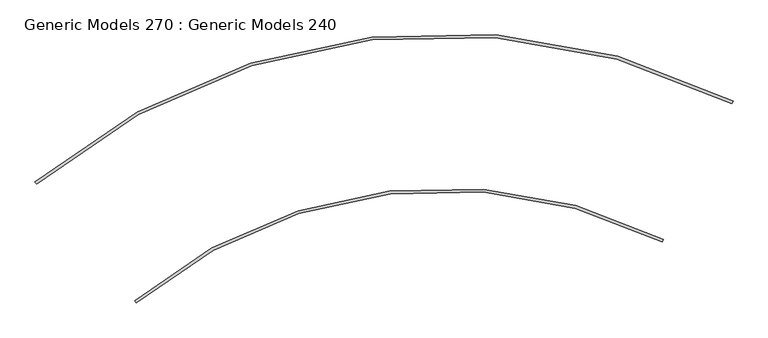
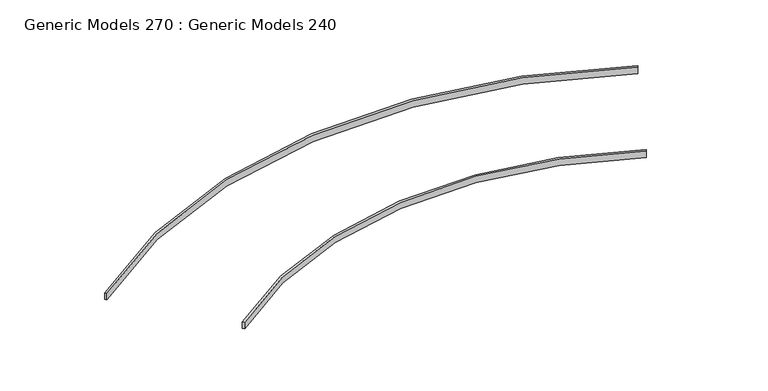
"""IFC4 building model written with IfcOpenShell, lengths in millimetres: proxy geometry, Generic Models 270 : Generic Models 240."""

from ifc_helpers import new_model, si_unit, point, frame, frame_2d, origin, place, context, project, spatial, polyline, circle_curve, trimmed, segment, composite_curve, outline, extrude, source, transform, mapped, element, save


def generic_models_270_generic_models_240_cf217300(model_context):
    return source(origin(), model_context, "Body", "SweptSolid", [
        extrude(outline(composite_curve([segment(trimmed(circle_curve(frame_2d((-832.04683, -25139.2753781)), 2232.5947981), [point((-2265.0114479, -23427.2321729))], [point((170.1471162, -23144.2598827))], False, "CARTESIAN"), True, "CONTINUOUS"), segment(polyline([(170.1471162, -23144.2598827), (164.4461878, -23155.6084251)]), True, "CONTINUOUS"), segment(trimmed(circle_curve(frame_2d((-832.04683, -25139.2753781)), 2219.8947981), [point((164.4461878, -23155.6084251))], [point((-2256.8601028, -23436.9710421))], True, "CARTESIAN"), True, "CONTINUOUS"), segment(polyline([(-2256.8601028, -23436.9710421), (-2265.0114479, -23427.2321729)]), True, "CONTINUOUS")], self_intersect=False)), frame((0.0, 0.0, 781.05), z_axis=(0.0, 0.0, 1.0), x_axis=(1.0, 0.0, 0.0)), (0.0, 0.0, 1.0), 38.1),
        extrude(outline(composite_curve([segment(trimmed(circle_curve(frame_2d((-832.04683, -25139.2753781)), 2947.0118053), [point((-2723.5515711, -22879.3885678))], [point((490.8431961, -22505.8668341))], False, "CARTESIAN"), True, "CONTINUOUS"), segment(polyline([(490.8431961, -22505.8668341), (485.1422677, -22517.2153765)]), True, "CONTINUOUS"), segment(trimmed(circle_curve(frame_2d((-832.04683, -25139.2753781)), 2934.3118053), [point((485.1422677, -22517.2153765))], [point((-2715.400226, -22889.127437))], True, "CARTESIAN"), True, "CONTINUOUS"), segment(polyline([(-2715.400226, -22889.127437), (-2723.5515711, -22879.3885678)]), True, "CONTINUOUS")], self_intersect=False)), frame((0.0, 0.0, 781.05), z_axis=(0.0, 0.0, 1.0), x_axis=(1.0, 0.0, 0.0)), (0.0, 0.0, 1.0), 38.1),
    ])


if __name__ == "__main__":
    model = new_model("IFC4")
    model_context = context("Model", 3, world=origin())
    ifc_project = project(units=[si_unit("LENGTHUNIT", "METRE", prefix="MILLI")], contexts=[model_context])
    site = spatial("IfcSite", under=ifc_project)
    building = spatial("IfcBuilding", under=site)
    placement = place(None, origin())
    generic_models_270_generic_models_240_shape = generic_models_270_generic_models_240_cf217300(model_context)
    element("IfcBuildingElementProxy", 1, Name="Generic Models 270 : Generic Models 240", ObjectType="Generic Models 270 : Generic Models 240", at=placement, inside=building, context=model_context, shape_type="MappedRepresentation", body=[
        mapped(generic_models_270_generic_models_240_shape, transform((0.0, 0.0, 0.0), x_axis=(1.0, 0.0, 0.0), y_axis=(0.0, 1.0, 0.0), z_axis=(0.0, 0.0, 1.0))),
    ])
    save(model, "model.ifc")

# Revit data of these elements
# Element 1 (IfcBuildingElementProxy, "Generic Models 270 : Generic Models 240")
#   Materials on its faces: "1/2\" x 2\" TRIM BOARD"
# Materials
#   "1/2\" x 2\" TRIM BOARD": class "Wood", colour RGB 48 37 22, transparency 0, Description = "Pinus Echinata", Cost = 0
